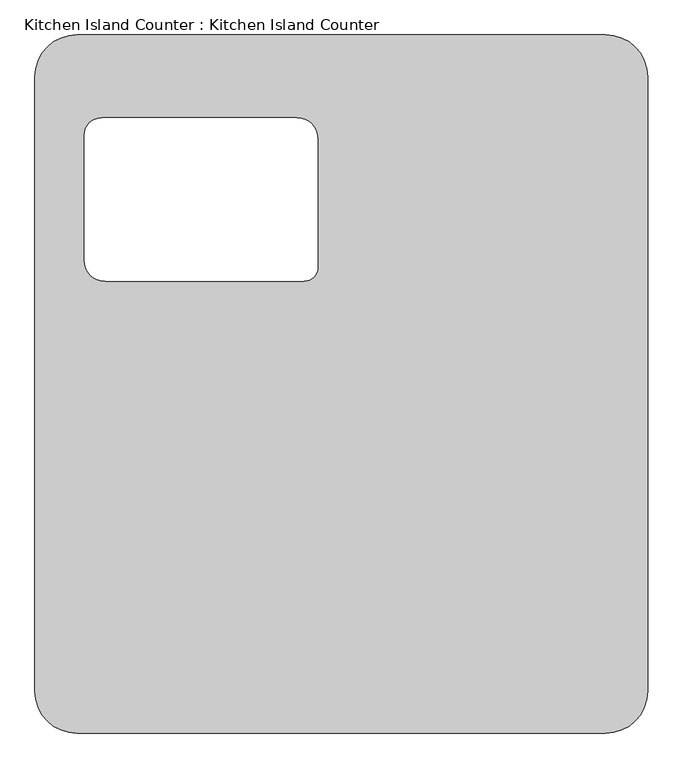
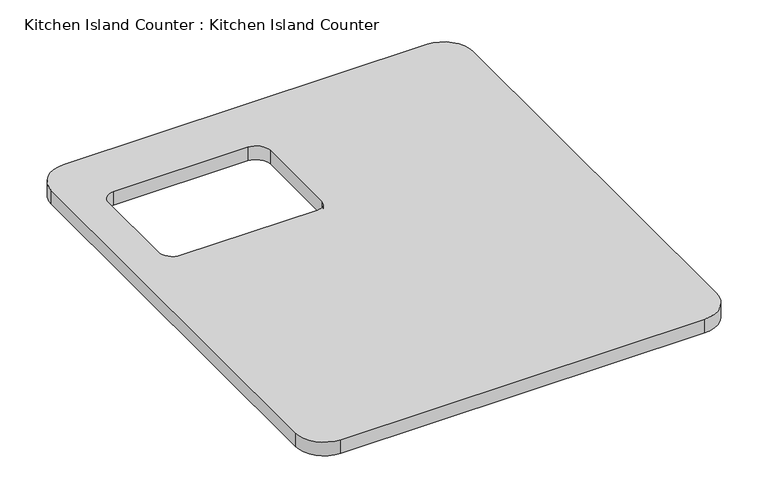
"""IFC4 building model written with IfcOpenShell, lengths in millimetres: furniture geometry, Kitchen Island Counter : Kitchen Island Counter."""

from ifc_helpers import new_model, si_unit, point, frame, frame_2d, origin, place, context, project, spatial, polyline, circle_curve, trimmed, segment, composite_curve, outline, extrude, source, transform, mapped, element, save


def kitchen_island_counter_kitchen_island_counter_32e57820(model_context):
    return source(origin(), model_context, "Body", "SweptSolid", [
        extrude(outline(composite_curve([segment(trimmed(circle_curve(frame_2d((6537.1738446, 11622.0875)), 76.2), [point((6537.1738446, 11698.2875))], [point((6613.3738446, 11622.0875))], False, "CARTESIAN"), True, "CONTINUOUS"), segment(polyline([(6613.3738446, 11622.0875), (6613.3738446, 10500.9991254)]), True, "CONTINUOUS"), segment(trimmed(circle_curve(frame_2d((6537.1738446, 10500.9991254)), 76.2), [point((6613.3738446, 10500.9991254))], [point((6537.1738446, 10424.7991254))], False, "CARTESIAN"), True, "CONTINUOUS"), segment(polyline([(6537.1738446, 10424.7991254), (5571.9738446, 10424.7991254)]), True, "CONTINUOUS"), segment(trimmed(circle_curve(frame_2d((5571.9738446, 10500.9991254)), 76.2), [point((5571.9738446, 10424.7991254))], [point((5495.7738446, 10500.9991254))], False, "CARTESIAN"), True, "CONTINUOUS"), segment(polyline([(5495.7738446, 10500.9991254), (5495.7738446, 11622.0875)]), True, "CONTINUOUS"), segment(trimmed(circle_curve(frame_2d((5571.9738446, 11622.0875)), 76.2), [point((5495.7738446, 11622.0875))], [point((5571.9738446, 11698.2875))], False, "CARTESIAN"), True, "CONTINUOUS"), segment(polyline([(5571.9738446, 11698.2875), (6537.1738446, 11698.2875)]), True, "CONTINUOUS")], self_intersect=False), holes=[composite_curve([segment(trimmed(circle_curve(frame_2d((5623.7298741, 11287.2510244)), 38.1), [point((5585.6298741, 11287.2510244))], [point((5623.7298741, 11249.1510244))], True, "CARTESIAN"), True, "CONTINUOUS"), segment(polyline([(5623.7298741, 11249.1510244), (5986.463181, 11249.1510244)]), True, "CONTINUOUS"), segment(trimmed(circle_curve(frame_2d((5986.463181, 11274.5510244)), 25.4), [point((5986.463181, 11249.1510244))], [point((6011.863181, 11274.5510244))], True, "CARTESIAN"), True, "CONTINUOUS"), segment(polyline([(6011.863181, 11274.5510244), (6011.863181, 11508.987199)]), True, "CONTINUOUS"), segment(trimmed(circle_curve(frame_2d((5973.763181, 11508.987199)), 38.1), [point((6011.863181, 11508.987199))], [point((5973.763181, 11547.087199))], True, "CARTESIAN"), True, "CONTINUOUS"), segment(polyline([(5973.763181, 11547.087199), (5617.3798741, 11547.087199)]), True, "CONTINUOUS"), segment(trimmed(circle_curve(frame_2d((5617.3798741, 11515.337199)), 31.75), [point((5617.3798741, 11547.087199))], [point((5585.6298741, 11515.337199))], True, "CARTESIAN"), True, "CONTINUOUS"), segment(polyline([(5585.6298741, 11515.337199), (5585.6298741, 11287.2510244)]), True, "CONTINUOUS")], self_intersect=False)]), frame((0.0, 0.0, 876.3), z_axis=(0.0, 0.0, 1.0), x_axis=(1.0, 0.0, 0.0)), (0.0, 0.0, 1.0), 38.1),
    ])


if __name__ == "__main__":
    model = new_model("IFC4")
    model_context = context("Model", 3, world=origin())
    ifc_project = project(units=[si_unit("LENGTHUNIT", "METRE", prefix="MILLI")], contexts=[model_context])
    site = spatial("IfcSite", under=ifc_project)
    building = spatial("IfcBuilding", under=site)
    placement = place(None, origin())
    kitchen_island_counter_kitchen_island_counter_shape = kitchen_island_counter_kitchen_island_counter_32e57820(model_context)
    element("IfcFurniture", 1, ObjectType="Kitchen Island Counter : Kitchen Island Counter", at=placement, inside=building, context=model_context, shape_type="MappedRepresentation", body=[
        mapped(kitchen_island_counter_kitchen_island_counter_shape, transform((0.0, 0.0, 0.0), x_axis=(1.0, 0.0, 0.0), y_axis=(0.0, 1.0, 0.0), z_axis=(0.0, 0.0, 1.0))),
    ])
    save(model, "model.ifc")

# Revit data of these elements
# Type "Kitchen Island Counter : Kitchen Island Counter"
#   COBie.Type = no
# Element 1 (IfcFurniture, "Kitchen Island Counter : Kitchen Island Counter")
#   Materials on its faces: "Corian - Dusk"
# Materials
#   "Corian - Dusk": class "Plastic", colour RGB 75 95 146, transparency 0, Manufacturer = "Corning", Cost = 0
